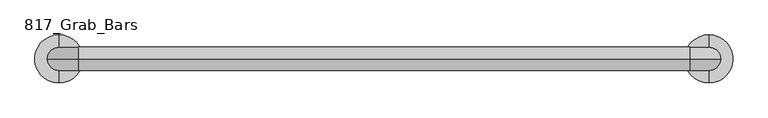
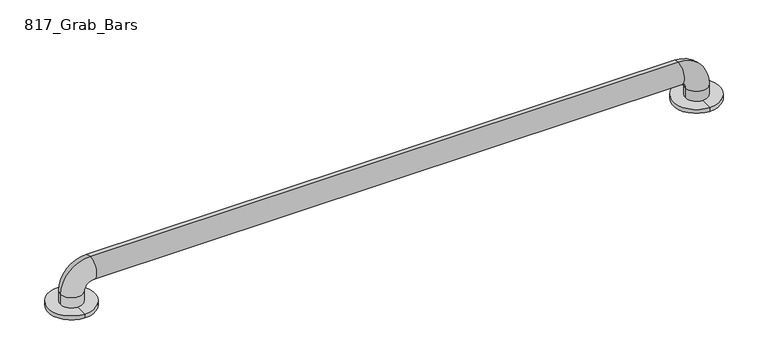
"""IFC4 building model written with IfcOpenShell, lengths in millimetres: proxy geometry, 817_Grab_Bars : 8170-001420."""

import ifcopenshell
import ifcopenshell.guid

model = None  # the IFC model being written
_history = None  # IfcOwnerHistory: only IFC2X3 demands one
_inside = {}  # id of a spatial element -> (the spatial element, [elements in it])
_under = {}  # id of a project, library or spatial element -> (it, [spatial elements below it])
_declared = {}  # id of a project -> (the project, [libraries it declares])
_typed = {}  # id of a type object -> (the type object, [elements of that type])
_made_of = {}  # id of a material, layer set ... -> (it, [elements and type objects made of it])


def new_model(schema):
    """Start an empty IFC model of exactly this schema.

    Asked for "IFC4X3", IfcOpenShell would pick the latest addendum, in which some entities
    have other attributes; the version numbers below select the first issue.
    IFC2X3 requires an IfcOwnerHistory on every rooted entity: one is made here for all.
    """
    global model, _history
    if schema == "IFC4X3":
        model = ifcopenshell.file(schema_version=(4, 3, 0, 0))
    else:
        model = ifcopenshell.file(schema=schema)
    _inside.clear()
    _under.clear()
    _declared.clear()
    _typed.clear()
    _made_of.clear()
    _history = None
    if model.schema == "IFC2X3":
        org = make("IfcOrganization", Name="unknown")
        user = make(
            "IfcPersonAndOrganization",
            ThePerson=make("IfcPerson", FamilyName="unknown"),
            TheOrganization=org,
        )
        app = make(
            "IfcApplication",
            ApplicationDeveloper=org,
            Version="unknown",
            ApplicationFullName="unknown",
            ApplicationIdentifier="unknown",
        )
        _history = make(
            "IfcOwnerHistory",
            OwningUser=user,
            OwningApplication=app,
            ChangeAction="ADDED",
            CreationDate=0,
        )
    return model


def make(cls, **values):
    """One entity of the class cls with the attributes given. An attribute that is None is left unset."""
    return model.create_entity(
        cls, **{name: value for name, value in values.items() if value is not None}
    )


def rooted(cls, **values):
    """An entity with a GlobalId (a new one), such as an element, a storey or a relation."""
    return make(cls, GlobalId=ifcopenshell.guid.new(), OwnerHistory=_history, **values)


def si_unit(unit_type, name, prefix=None):
    """IfcSIUnit, for example si_unit("LENGTHUNIT", "METRE", prefix="MILLI")."""
    return make("IfcSIUnit", UnitType=unit_type, Prefix=prefix, Name=name)


def assignment(units):
    """IfcUnitAssignment: the units of a project."""
    return None if units is None else make("IfcUnitAssignment", Units=units)


def point(xyz):
    """IfcCartesianPoint."""
    return None if xyz is None else make("IfcCartesianPoint", Coordinates=xyz)


def direction(xyz):
    """IfcDirection."""
    return None if xyz is None else make("IfcDirection", DirectionRatios=xyz)


def frame(location, z_axis=None, x_axis=None):
    """IfcAxis2Placement3D, a coordinate frame: its origin and axes. An axis left out is left unset."""
    return make(
        "IfcAxis2Placement3D",
        Location=point(location),
        Axis=direction(z_axis),
        RefDirection=direction(x_axis),
    )


def origin():
    """The frame at (0, 0, 0) with its axes left unset."""
    return frame((0.0, 0.0, 0.0))


def place(relative_to, where):
    """IfcLocalPlacement: puts the frame where relative to a parent placement (None: the world)."""
    return make(
        "IfcLocalPlacement", PlacementRelTo=relative_to, RelativePlacement=where
    )


def context(
    kind, dimensions, precision=None, world=None, true_north=None, identifier=None
):
    """IfcGeometricRepresentationContext, for example the 3D "Model" context."""
    return make(
        "IfcGeometricRepresentationContext",
        ContextIdentifier=identifier,
        ContextType=kind,
        CoordinateSpaceDimension=dimensions,
        Precision=precision,
        WorldCoordinateSystem=world,
        TrueNorth=true_north,
    )


def project(units=None, contexts=None):
    """IfcProject with its units and contexts."""
    return rooted(
        "IfcProject",
        Name="project",
        RepresentationContexts=contexts,
        UnitsInContext=assignment(units),
    )


def spatial(cls, under=None, at=None, **own):
    """A site, building, storey or space (cls), placed at a placement, below another one or the project."""
    s = rooted(cls, ObjectPlacement=at, **own)
    if under is not None:
        _under.setdefault(under.id(), (under, []))[1].append(s)
    return s


def circle_curve(where, radius):
    """IfcCircle in the frame where."""
    return make("IfcCircle", Position=where, Radius=radius)


def ellipse_curve(where, semi_axis1, semi_axis2):
    """IfcEllipse in the frame where."""
    return make(
        "IfcEllipse", Position=where, SemiAxis1=semi_axis1, SemiAxis2=semi_axis2
    )


def trimmed(basis, trim1, trim2, sense, master):
    """IfcTrimmedCurve: the piece of a basis curve between two trims."""
    return make(
        "IfcTrimmedCurve",
        BasisCurve=basis,
        Trim1=trim1,
        Trim2=trim2,
        SenseAgreement=sense,
        MasterRepresentation=master,
    )


def shape(context_of_items, identifier, shape_type, items):
    """IfcShapeRepresentation: the items that make up one representation, for example the "Body"."""
    return make(
        "IfcShapeRepresentation",
        ContextOfItems=context_of_items,
        RepresentationIdentifier=identifier,
        RepresentationType=shape_type,
        Items=items,
    )


def source(mapping_origin, context_of_items, identifier, shape_type, items):
    """IfcRepresentationMap: a shape defined once, which mapped items show again and again."""
    return make(
        "IfcRepresentationMap",
        MappingOrigin=mapping_origin,
        MappedRepresentation=shape(context_of_items, identifier, shape_type, items),
    )


def transform(
    local_origin,
    x_axis=None,
    y_axis=None,
    z_axis=None,
    scale=None,
    scale2=None,
    scale3=None,
    uniform=True,
):
    """IfcCartesianTransformationOperator3D, or its non-uniform kind. x_axis, y_axis, z_axis: its Axis1, 2, 3."""
    if uniform:
        return make(
            "IfcCartesianTransformationOperator3D",
            Axis1=direction(x_axis),
            Axis2=direction(y_axis),
            LocalOrigin=point(local_origin),
            Scale=scale,
            Axis3=direction(z_axis),
        )
    return make(
        "IfcCartesianTransformationOperator3DnonUniform",
        Axis1=direction(x_axis),
        Axis2=direction(y_axis),
        LocalOrigin=point(local_origin),
        Scale=scale,
        Axis3=direction(z_axis),
        Scale2=scale2,
        Scale3=scale3,
    )


def mapped(mapping_source, mapping_target):
    """IfcMappedItem: shows the shape of a source again, moved by a transform."""
    return make(
        "IfcMappedItem", MappingSource=mapping_source, MappingTarget=mapping_target
    )


def made_of(thing, what):
    """Note that an element or type object is made of a material, layer set ...; save() writes the relation."""
    if what is not None:
        _made_of.setdefault(what.id(), (what, []))[1].append(thing)
    return thing


def element(
    cls,
    number,
    at=None,
    inside=None,
    cuts=None,
    type_object=None,
    material=None,
    context=None,
    identifier="Body",
    shape_type=None,
    held_by="IfcProductDefinitionShape",
    body=None,
    shapes=None,
    **own,
):
    """One element of the class cls, such as IfcWall. Its Tag is "e" and its number.

    at: its placement. inside: the storey or other place that contains it. cuts: it is an
    opening in that element (IfcRelVoidsElement). A single representation is given by context,
    identifier, shape_type and body (its items); several are given by shapes. held_by: the class
    of the entity that holds the representations. save() writes the other relations.
    """
    e = rooted(cls, Tag="e%d" % number, ObjectPlacement=at, **own)
    if body is not None:
        shapes = [shape(context, identifier, shape_type, body)]
    if shapes is not None:
        e.Representation = make(held_by, Representations=shapes)
    if inside is not None:
        _inside.setdefault(inside.id(), (inside, []))[1].append(e)
    if cuts is not None:
        rooted(
            "IfcRelVoidsElement", RelatingBuildingElement=cuts, RelatedOpeningElement=e
        )
    if type_object is not None:
        _typed.setdefault(type_object.id(), (type_object, []))[1].append(e)
    return made_of(e, material)


def aggregate(whole, parts):
    """IfcRelAggregates: a whole, such as a stair, and the parts it consists of."""
    return rooted("IfcRelAggregates", RelatingObject=whole, RelatedObjects=parts)


def save(model, path):
    """Write the relations noted so far, then the file.

    IfcRelAggregates (storeys below a building ...), IfcRelContainedInSpatialStructure (elements
    in a storey), IfcRelDefinesByType, IfcRelAssociatesMaterial and IfcRelDeclares: one each for
    every whole, place, type object, material and project.
    """
    for whole, parts in _under.values():
        aggregate(whole, parts)
    for where, things in _inside.values():
        rooted(
            "IfcRelContainedInSpatialStructure",
            RelatedElements=things,
            RelatingStructure=where,
        )
    for kind, things in _typed.values():
        rooted("IfcRelDefinesByType", RelatedObjects=things, RelatingType=kind)
    for what, things in _made_of.values():
        rooted("IfcRelAssociatesMaterial", RelatedObjects=things, RelatingMaterial=what)
    for by, libraries in _declared.values():
        rooted("IfcRelDeclares", RelatingContext=by, RelatedDefinitions=libraries)
    model.write(path)


def plane_surface(at):
    """IfcPlane: the flat surface through the origin of the frame at, square to its z axis."""
    return make("IfcPlane", Position=at)


def cylinder_surface(at, radius):
    """IfcCylindricalSurface: all points at the distance radius from the z axis of the frame at."""
    return make("IfcCylindricalSurface", Position=at, Radius=radius)


def revolved_surface(curve, axis_point, axis_direction):
    """IfcSurfaceOfRevolution: the curve turned about the line through axis_point along axis_direction."""
    return make(
        "IfcSurfaceOfRevolution",
        SweptCurve=make("IfcArbitraryOpenProfileDef", ProfileType="CURVE", Curve=curve),
        AxisPosition=make("IfcAxis1Placement", Location=point(axis_point), Axis=direction(axis_direction)),
    )


def advanced_brep(points, edges, surfaces, faces):
    """IfcAdvancedBrep: a solid bounded by faces that lie on surfaces and meet in shared edges.

    An edge is (start, end): straight between two places in points (the first is 0);
    or (start, end, curve); or (start, end, curve, False) where it runs against its curve.
    A face is (place in surfaces, loops), or (place, loops, False) where it looks against
    its surface's normal. A loop lists edges by number (the first is 1), with a minus sign
    where the edge is run from its end to its start. The first loop is the outer one.
    """
    corners = [point(p) for p in points]
    vertices = [make("IfcVertexPoint", VertexGeometry=c) for c in corners]
    made = []
    for start, end, *more in edges:
        made.append(
            make(
                "IfcEdgeCurve",
                EdgeStart=vertices[start],
                EdgeEnd=vertices[end],
                EdgeGeometry=more[0] if more else make("IfcPolyline", Points=[corners[start], corners[end]]),
                SameSense=more[1] if len(more) > 1 else True,
            )
        )
    hull = []
    for where, loops, *sense in faces:
        bounds = []
        for j, loop in enumerate(loops):
            ring = [make("IfcOrientedEdge", EdgeElement=made[abs(k) - 1], Orientation=k > 0) for k in loop]
            bounds.append(
                make(
                    "IfcFaceOuterBound" if j == 0 else "IfcFaceBound",
                    Bound=make("IfcEdgeLoop", EdgeList=ring),
                    Orientation=True,
                )
            )
        hull.append(make("IfcAdvancedFace", Bounds=bounds, FaceSurface=surfaces[where], SameSense=sense[0] if sense else True))
    return make("IfcAdvancedBrep", Outer=make("IfcClosedShell", CfsFaces=hull))


def proxy_817_grab_bars_e388bd4b(model_context):
    return source(origin(), model_context, "Body", "AdvancedBrep", [
        advanced_brep(
        [(-439.7375, -496.8875, 7.14375), (-439.7375, -576.2625, 7.14375), (-439.7375, -555.625, 7.14375), (-458.7875, -536.575, 7.14375), (-439.7375, -517.525, 7.14375), (-420.6875, -536.575, 7.14375), (-439.7375, -576.2625, 0.0), (-439.7375, -496.8875, 0.0), (-439.7375, -517.525, 0.0), (-439.7375, -536.575, 0.0), (-439.7375, -555.625, 0.0), (627.0625, -496.8875, 7.14375), (627.0625, -576.2625, 7.14375), (627.0625, -555.625, 7.14375), (608.0125, -536.575, 7.14375), (627.0625, -517.525, 7.14375), (646.1125, -536.575, 7.14375), (627.0625, -576.2625, 0.0), (627.0625, -496.8875, 0.0), (627.0625, -517.525, 0.0), (627.0625, -536.575, 0.0), (627.0625, -555.625, 0.0), (-458.7875, -536.575, 25.4), (-420.6875, -536.575, 25.4), (-407.9875, -536.575, 76.2), (-407.9875, -536.575, 38.1), (595.3125, -536.575, 76.2), (595.3125, -536.575, 38.1), (646.1125, -536.575, 25.4), (608.0125, -536.575, 25.4)],
        [
            (0, 1, circle_curve(frame((-439.7375, -536.575, 7.14375), z_axis=(0.0, 0.0, 1.0), x_axis=(0.0, 1.0, 0.0)), 39.6875)),
            (1, 2),
            (2, 3, circle_curve(frame((-439.7375, -536.575, 7.14375), z_axis=(0.0, 0.0, -1.0), x_axis=(1.0, 0.0, 0.0)), 19.05)),
            (3, 4, circle_curve(frame((-439.7375, -536.575, 7.14375), z_axis=(0.0, 0.0, -1.0), x_axis=(1.0, 0.0, 0.0)), 19.05)),
            (4, 0),
            (1, 0, circle_curve(frame((-439.7375, -536.575, 7.14375), z_axis=(0.0, 0.0, 1.0), x_axis=(0.0, 1.0, 0.0)), 39.6875)),
            (4, 5, circle_curve(frame((-439.7375, -536.575, 7.14375), z_axis=(0.0, 0.0, -1.0), x_axis=(1.0, 0.0, 0.0)), 19.05)),
            (5, 2, circle_curve(frame((-439.7375, -536.575, 7.14375), z_axis=(0.0, 0.0, -1.0), x_axis=(1.0, 0.0, 0.0)), 19.05)),
            (6, 7, circle_curve(frame((-439.7375, -536.575, 0.0), z_axis=(0.0, 0.0, -1.0), x_axis=(0.0, 1.0, 0.0)), 39.6875)),
            (7, 8),
            (8, 9),
            (9, 10),
            (10, 6),
            (7, 6, circle_curve(frame((-439.7375, -536.575, 0.0), z_axis=(0.0, 0.0, -1.0), x_axis=(0.0, 1.0, 0.0)), 39.6875)),
            (0, 7),
            (6, 1),
            (11, 12, circle_curve(frame((627.0625, -536.575, 7.14375), z_axis=(0.0, 0.0, 1.0), x_axis=(0.0, 1.0, 0.0)), 39.6875)),
            (12, 13),
            (13, 14, circle_curve(frame((627.0625, -536.575, 7.14375), z_axis=(0.0, 0.0, -1.0), x_axis=(-1.0, 0.0, 0.0)), 19.05)),
            (14, 15, circle_curve(frame((627.0625, -536.575, 7.14375), z_axis=(0.0, 0.0, -1.0), x_axis=(-1.0, 0.0, 0.0)), 19.05)),
            (15, 11),
            (12, 11, circle_curve(frame((627.0625, -536.575, 7.14375), z_axis=(0.0, 0.0, 1.0), x_axis=(0.0, 1.0, 0.0)), 39.6875)),
            (15, 16, circle_curve(frame((627.0625, -536.575, 7.14375), z_axis=(0.0, 0.0, -1.0), x_axis=(-1.0, 0.0, 0.0)), 19.05)),
            (16, 13, circle_curve(frame((627.0625, -536.575, 7.14375), z_axis=(0.0, 0.0, -1.0), x_axis=(-1.0, 0.0, 0.0)), 19.05)),
            (17, 18, circle_curve(frame((627.0625, -536.575, 0.0), z_axis=(0.0, 0.0, -1.0), x_axis=(0.0, 1.0, 0.0)), 39.6875)),
            (18, 19),
            (19, 20),
            (20, 21),
            (21, 17),
            (18, 17, circle_curve(frame((627.0625, -536.575, 0.0), z_axis=(0.0, 0.0, -1.0), x_axis=(0.0, 1.0, 0.0)), 39.6875)),
            (11, 18),
            (17, 12),
            (22, 23, circle_curve(frame((-439.7375, -536.575, 25.4), z_axis=(0.0, 0.0, -1.0), x_axis=(1.0, 0.0, 0.0)), 19.05)),
            (23, 5),
            (3, 22),
            (23, 22, circle_curve(frame((-439.7375, -536.575, 25.4), z_axis=(0.0, 0.0, -1.0), x_axis=(1.0, 0.0, 0.0)), 19.05)),
            (22, 24, circle_curve(frame((-407.9875, -536.575, 25.4), z_axis=(0.0, 1.0, 0.0), x_axis=(-1.0, 0.0, 0.0)), 50.8)),
            (24, 25, circle_curve(frame((-407.9875, -536.575, 57.15), z_axis=(-1.0, 0.0, 0.0), x_axis=(0.0, 0.0, -1.0)), 19.05)),
            (25, 23, circle_curve(frame((-407.9875, -536.575, 25.4), z_axis=(0.0, -1.0, 0.0), x_axis=(-1.0, 0.0, 0.0)), 12.7)),
            (25, 24, circle_curve(frame((-407.9875, -536.575, 57.15), z_axis=(-1.0, 0.0, 0.0), x_axis=(0.0, 0.0, -1.0)), 19.05)),
            (24, 26),
            (26, 27, circle_curve(frame((595.3125, -536.575, 57.15), z_axis=(-1.0, 0.0, 0.0), x_axis=(0.0, 0.0, -1.0)), 19.05)),
            (27, 25),
            (27, 26, circle_curve(frame((595.3125, -536.575, 57.15), z_axis=(-1.0, 0.0, 0.0), x_axis=(0.0, 0.0, -1.0)), 19.05)),
            (26, 28, circle_curve(frame((595.3125, -536.575, 25.4), z_axis=(0.0, 1.0, 0.0), x_axis=(0.0, 0.0, 1.0)), 50.8)),
            (28, 29, circle_curve(frame((627.0625, -536.575, 25.4), z_axis=(0.0, 0.0, 1.0), x_axis=(-1.0, 0.0, 0.0)), 19.05)),
            (29, 27, circle_curve(frame((595.3125, -536.575, 25.4), z_axis=(0.0, -1.0, 0.0), x_axis=(0.0, 0.0, 1.0)), 12.7)),
            (29, 28, circle_curve(frame((627.0625, -536.575, 25.4), z_axis=(0.0, 0.0, 1.0), x_axis=(-1.0, 0.0, 0.0)), 19.05)),
            (28, 16),
            (14, 29),
        ],
        [
            plane_surface(frame((-439.7375, -536.575, 7.14375), z_axis=(0.0, 0.0, 1.0), x_axis=(0.0, 1.0, 0.0))),
            plane_surface(frame((-439.7375, -536.575, 0.0), z_axis=(0.0, 0.0, -1.0), x_axis=(0.0, 1.0, 0.0))),
            cylinder_surface(frame((-439.7375, -536.575, 7.14375), z_axis=(0.0, 0.0, 1.0), x_axis=(0.0, 1.0, 0.0)), 39.6875),
            plane_surface(frame((627.0625, -536.575, 7.14375), z_axis=(0.0, 0.0, 1.0), x_axis=(0.0, 1.0, 0.0))),
            plane_surface(frame((627.0625, -536.575, 0.0), z_axis=(0.0, 0.0, -1.0), x_axis=(0.0, 1.0, 0.0))),
            cylinder_surface(frame((627.0625, -536.575, 31.75), z_axis=(0.0, 0.0, 1.0), x_axis=(0.0, 1.0, 0.0)), 39.6875),
            cylinder_surface(frame((-439.7375, -536.575, 0.0), z_axis=(0.0, 0.0, -1.0), x_axis=(1.0, 0.0, 0.0)), 19.05),
            revolved_surface(trimmed(ellipse_curve(frame((-439.7375, -536.575, 25.4), z_axis=(0.0, 0.0, -1.0), x_axis=(1.0, 0.0, 0.0)), 19.05, 19.05), [point((-458.7875, -536.575, 25.4))], [point((-420.6875, -536.575, 25.4))], True, "CARTESIAN"), (-407.9875, -536.575, 25.4), (0.0, 1.0, 0.0)),
            revolved_surface(trimmed(ellipse_curve(frame((-439.7375, -536.575, 25.4), z_axis=(0.0, 0.0, -1.0), x_axis=(1.0, 0.0, 0.0)), 19.05, 19.05), [point((-420.6875, -536.575, 25.4))], [point((-458.7875, -536.575, 25.4))], True, "CARTESIAN"), (-407.9875, -536.575, 25.4), (0.0, 1.0, 0.0)),
            cylinder_surface(frame((-407.9875, -536.575, 57.15), z_axis=(-1.0, 0.0, 0.0), x_axis=(0.0, 0.0, -1.0)), 19.05),
            revolved_surface(trimmed(ellipse_curve(frame((595.3125, -536.575, 57.15), z_axis=(-1.0, 0.0, 0.0), x_axis=(0.0, 0.0, -1.0)), 19.05, 19.05), [point((595.3125, -536.575, 76.2))], [point((595.3125, -536.575, 38.1))], True, "CARTESIAN"), (595.3125, -536.575, 25.4), (0.0, 1.0, 0.0)),
            revolved_surface(trimmed(ellipse_curve(frame((595.3125, -536.575, 57.15), z_axis=(-1.0, 0.0, 0.0), x_axis=(0.0, 0.0, -1.0)), 19.05, 19.05), [point((595.3125, -536.575, 38.1))], [point((595.3125, -536.575, 76.2))], True, "CARTESIAN"), (595.3125, -536.575, 25.4), (0.0, 1.0, 0.0)),
            cylinder_surface(frame((627.0625, -536.575, 25.4), z_axis=(0.0, 0.0, 1.0), x_axis=(-1.0, 0.0, 0.0)), 19.05),
        ],
        [
            (0, [[1, 2, 3, 4, 5]]),
            (0, [[6, -5, 7, 8, -2]]),
            (1, [[9, 10, 11, 12, 13]]),
            (1, [[14, -13, -12, -11, -10]]),
            (2, [[-1, 15, -9, 16]]),
            (2, [[-6, -16, -14, -15]]),
            (3, [[17, 18, 19, 20, 21]]),
            (3, [[22, -21, 23, 24, -18]]),
            (4, [[25, 26, 27, 28, 29]]),
            (4, [[30, -29, -28, -27, -26]]),
            (5, [[-17, 31, -25, 32]]),
            (5, [[-22, -32, -30, -31]]),
            (6, [[33, 34, -7, -4, 35]]),
            (6, [[36, -35, -3, -8, -34]]),
            (7, [[-33, 37, 38, 39]]),
            (8, [[-36, -39, 40, -37]]),
            (9, [[-38, 41, 42, 43]]),
            (9, [[-40, -43, 44, -41]]),
            (10, [[-42, 45, 46, 47]]),
            (11, [[-44, -47, 48, -45]]),
            (12, [[-46, 49, -23, -20, 50]]),
            (12, [[-48, -50, -19, -24, -49]]),
        ],
    ),
    ])


if __name__ == "__main__":
    model = new_model("IFC4")
    model_context = context("Model", 3, world=origin())
    ifc_project = project(units=[si_unit("LENGTHUNIT", "METRE", prefix="MILLI")], contexts=[model_context])
    site = spatial("IfcSite", under=ifc_project)
    building = spatial("IfcBuilding", under=site)
    placement = place(None, origin())
    proxy_817_grab_bars_shape = proxy_817_grab_bars_e388bd4b(model_context)
    element("IfcBuildingElementProxy", 1, Name="817_Grab_Bars : 8170-001420", ObjectType="817_Grab_Bars : 8170-001420", at=placement, inside=building, context=model_context, shape_type="MappedRepresentation", body=[
        mapped(proxy_817_grab_bars_shape, transform((0.0, 0.0, 0.0), x_axis=(1.0, 0.0, 0.0), y_axis=(0.0, 1.0, 0.0), z_axis=(0.0, 0.0, 1.0))),
    ])
    save(model, "model.ifc")

# Revit data of these elements
# Type "817_Grab_Bars : 8170-001420"
#   Keynote = "M10281313.01"
#   Warranty Information = "Complete unit, one (1) year"
#   Version = "1.0"
#   Technical Data = "http://www.bradleycorp.com/products/techdata/8815.pdf"
#   URL = "www.bradleycorp.com"
#   Type Comments = "All grab bar configurations are specified using centerline to centerline dimensions."
#   OmniClass Title = ""
#   Modeling Code = ""
#   Model = "8170-001420"
#   Material Note = "FLANGES - 11 GA., TUBING - 18 GA."
#   MasterFormat Section Title = ""
#   Manufacturer = "Bradley Corporation"
#   LEED Credit = ""
#   Instructions [instance default] = "This is a face mounted fixture."
#   Industry Standards = "ANSI Standard A117.1, ADA, ABA, ADAAG, UFAS"
#   Fire Rating = "None"
#   Description = "Grab Bars"
#   Copyright = "This Model Data is Property of Bradley Corporation"
#   Complies to NAFTA = "Yes"
#   Complies To Buy American Act = "Yes"
#   Assembly Code = "C1030200"
#   ADA Compliant = "Yes"
#   Radius = 0' - 0 3/4"
#   Percentage of Recycled Content = 56.77
#   Overall Length = 3' - 9 1/8"
#   OmniClass Number = 0
#   MasterFormat Section Number = 0
#   Length = 3' - 6"
#   Diameter = 0' - 1 1/2"
#   Default Elevation = 2' - 9"
#   Material and Finish = Bradley Corp Stainless Steel - Satin
# Element 1 (IfcBuildingElementProxy, "817_Grab_Bars : 8170-001420")
#   Materials on its faces: "Bradley Corp Stainless Steel - Satin"
# Materials
#   "Bradley Corp Stainless Steel - Satin": class "Metal", colour RGB 189 187 185, transparency 0, Manufacturer = "Bradley Corporation", URL = "www.bradleycorp.com", Description = "Stainless Steel - Satin Finish", Cost = 0
